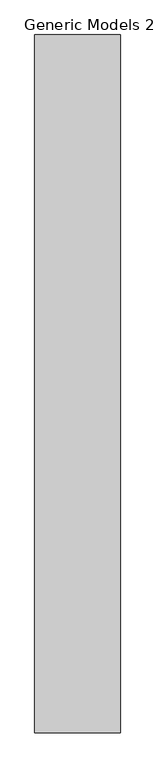
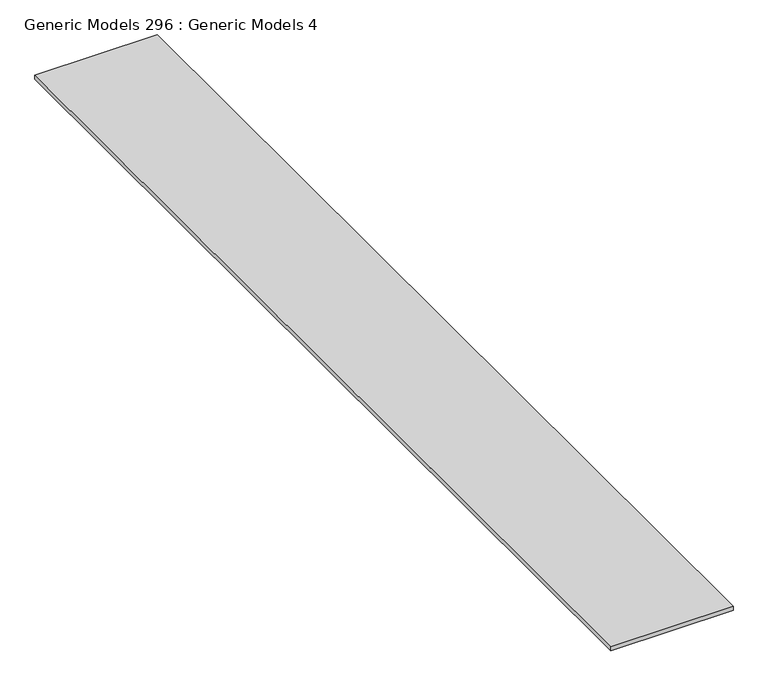
"""IFC4 building model written with IfcOpenShell, lengths in millimetres: proxy geometry, Generic Models 296 : Generic Models 4."""

from ifc_helpers import new_model, si_unit, frame, origin, place, context, project, spatial, polyline, outline, extrude, source, transform, mapped, element, save


def generic_models_296_generic_models_4_2ba87a2b(model_context):
    return source(origin(), model_context, "Body", "SweptSolid", [
        extrude(outline(polyline([(-5950.1236296, 2583.8769662), (-6498.6122941, 2583.8769662), (-6498.6122941, 7054.2769662), (-5950.1236296, 7054.2769662), (-5950.1236296, 2583.8769662)])), frame((0.0, 0.0, 123261.1835), z_axis=(0.0, 0.0, 1.0), x_axis=(1.0, 0.0, 0.0)), (0.0, 0.0, 1.0), 17.4625),
    ])


if __name__ == "__main__":
    model = new_model("IFC4")
    model_context = context("Model", 3, world=origin())
    ifc_project = project(units=[si_unit("LENGTHUNIT", "METRE", prefix="MILLI")], contexts=[model_context])
    site = spatial("IfcSite", under=ifc_project)
    building = spatial("IfcBuilding", under=site)
    placement = place(None, origin())
    generic_models_296_generic_models_4_shape = generic_models_296_generic_models_4_2ba87a2b(model_context)
    element("IfcBuildingElementProxy", 1, Name="Generic Models 296 : Generic Models 4", ObjectType="Generic Models 296 : Generic Models 4", at=placement, inside=building, context=model_context, shape_type="MappedRepresentation", body=[
        mapped(generic_models_296_generic_models_4_shape, transform((0.0, 0.0, 0.0), x_axis=(1.0, 0.0, 0.0), y_axis=(0.0, 1.0, 0.0), z_axis=(0.0, 0.0, 1.0))),
    ])
    save(model, "model.ifc")

# Revit data of these elements
# Element 1 (IfcBuildingElementProxy, "Generic Models 296 : Generic Models 4")
#   Materials on its faces: "_CDX PLYWOOD -  SEE STRUCT DWGs"
# Materials
#   "_CDX PLYWOOD -  SEE STRUCT DWGs": class "Generic", colour RGB 98 75 74, transparency 0, Cost = 0
